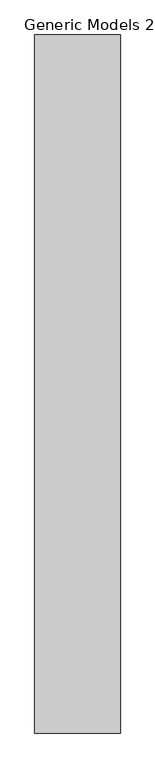
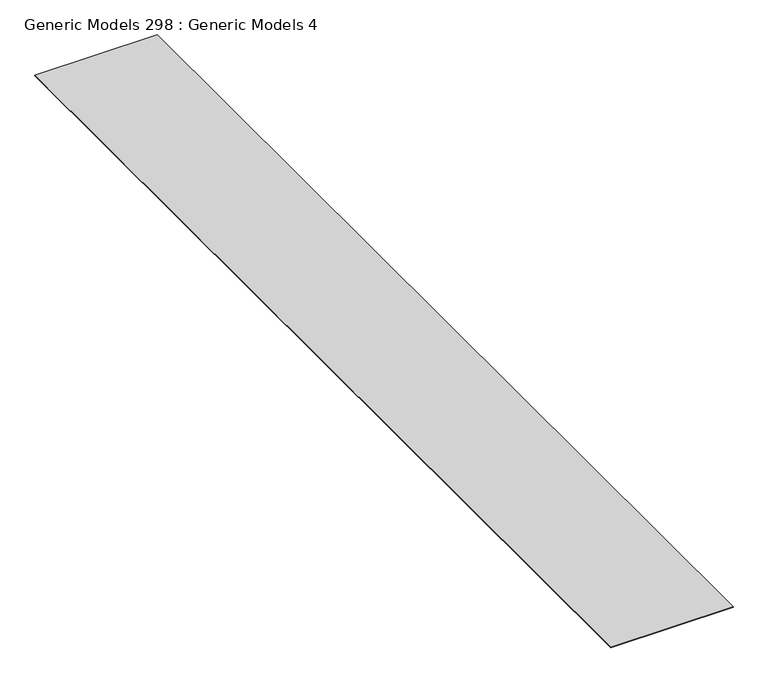
"""IFC4 building model written with IfcOpenShell, lengths in millimetres: proxy geometry, Generic Models 298 : Generic Models 4."""

import ifcopenshell
import ifcopenshell.guid

model = None  # the IFC model being written
_history = None  # IfcOwnerHistory: only IFC2X3 demands one
_inside = {}  # id of a spatial element -> (the spatial element, [elements in it])
_under = {}  # id of a project, library or spatial element -> (it, [spatial elements below it])
_declared = {}  # id of a project -> (the project, [libraries it declares])
_typed = {}  # id of a type object -> (the type object, [elements of that type])
_made_of = {}  # id of a material, layer set ... -> (it, [elements and type objects made of it])


def new_model(schema):
    """Start an empty IFC model of exactly this schema.

    Asked for "IFC4X3", IfcOpenShell would pick the latest addendum, in which some entities
    have other attributes; the version numbers below select the first issue.
    IFC2X3 requires an IfcOwnerHistory on every rooted entity: one is made here for all.
    """
    global model, _history
    if schema == "IFC4X3":
        model = ifcopenshell.file(schema_version=(4, 3, 0, 0))
    else:
        model = ifcopenshell.file(schema=schema)
    _inside.clear()
    _under.clear()
    _declared.clear()
    _typed.clear()
    _made_of.clear()
    _history = None
    if model.schema == "IFC2X3":
        org = make("IfcOrganization", Name="unknown")
        user = make(
            "IfcPersonAndOrganization",
            ThePerson=make("IfcPerson", FamilyName="unknown"),
            TheOrganization=org,
        )
        app = make(
            "IfcApplication",
            ApplicationDeveloper=org,
            Version="unknown",
            ApplicationFullName="unknown",
            ApplicationIdentifier="unknown",
        )
        _history = make(
            "IfcOwnerHistory",
            OwningUser=user,
            OwningApplication=app,
            ChangeAction="ADDED",
            CreationDate=0,
        )
    return model


def make(cls, **values):
    """One entity of the class cls with the attributes given. An attribute that is None is left unset."""
    return model.create_entity(
        cls, **{name: value for name, value in values.items() if value is not None}
    )


def rooted(cls, **values):
    """An entity with a GlobalId (a new one), such as an element, a storey or a relation."""
    return make(cls, GlobalId=ifcopenshell.guid.new(), OwnerHistory=_history, **values)


def si_unit(unit_type, name, prefix=None):
    """IfcSIUnit, for example si_unit("LENGTHUNIT", "METRE", prefix="MILLI")."""
    return make("IfcSIUnit", UnitType=unit_type, Prefix=prefix, Name=name)


def assignment(units):
    """IfcUnitAssignment: the units of a project."""
    return None if units is None else make("IfcUnitAssignment", Units=units)


def point(xyz):
    """IfcCartesianPoint."""
    return None if xyz is None else make("IfcCartesianPoint", Coordinates=xyz)


def direction(xyz):
    """IfcDirection."""
    return None if xyz is None else make("IfcDirection", DirectionRatios=xyz)


def frame(location, z_axis=None, x_axis=None):
    """IfcAxis2Placement3D, a coordinate frame: its origin and axes. An axis left out is left unset."""
    return make(
        "IfcAxis2Placement3D",
        Location=point(location),
        Axis=direction(z_axis),
        RefDirection=direction(x_axis),
    )


def origin():
    """The frame at (0, 0, 0) with its axes left unset."""
    return frame((0.0, 0.0, 0.0))


def place(relative_to, where):
    """IfcLocalPlacement: puts the frame where relative to a parent placement (None: the world)."""
    return make(
        "IfcLocalPlacement", PlacementRelTo=relative_to, RelativePlacement=where
    )


def context(
    kind, dimensions, precision=None, world=None, true_north=None, identifier=None
):
    """IfcGeometricRepresentationContext, for example the 3D "Model" context."""
    return make(
        "IfcGeometricRepresentationContext",
        ContextIdentifier=identifier,
        ContextType=kind,
        CoordinateSpaceDimension=dimensions,
        Precision=precision,
        WorldCoordinateSystem=world,
        TrueNorth=true_north,
    )


def project(units=None, contexts=None):
    """IfcProject with its units and contexts."""
    return rooted(
        "IfcProject",
        Name="project",
        RepresentationContexts=contexts,
        UnitsInContext=assignment(units),
    )


def spatial(cls, under=None, at=None, **own):
    """A site, building, storey or space (cls), placed at a placement, below another one or the project."""
    s = rooted(cls, ObjectPlacement=at, **own)
    if under is not None:
        _under.setdefault(under.id(), (under, []))[1].append(s)
    return s


def polyline(points):
    """IfcPolyline through the points."""
    return make("IfcPolyline", Points=[point(p) for p in points])


def outline(outer, holes=None, kind="AREA"):
    """IfcArbitraryClosedProfileDef: a profile drawn as a closed curve; with holes, ...WithVoids."""
    if holes is None:
        return make("IfcArbitraryClosedProfileDef", ProfileType=kind, OuterCurve=outer)
    return make(
        "IfcArbitraryProfileDefWithVoids",
        ProfileType=kind,
        OuterCurve=outer,
        InnerCurves=holes,
    )


def extrude(swept, where, along, depth):
    """IfcExtrudedAreaSolid: the profile swept, set in the frame where, extruded along a direction by depth."""
    return make(
        "IfcExtrudedAreaSolid",
        SweptArea=swept,
        Position=where,
        ExtrudedDirection=direction(along),
        Depth=depth,
    )


def shape(context_of_items, identifier, shape_type, items):
    """IfcShapeRepresentation: the items that make up one representation, for example the "Body"."""
    return make(
        "IfcShapeRepresentation",
        ContextOfItems=context_of_items,
        RepresentationIdentifier=identifier,
        RepresentationType=shape_type,
        Items=items,
    )


def source(mapping_origin, context_of_items, identifier, shape_type, items):
    """IfcRepresentationMap: a shape defined once, which mapped items show again and again."""
    return make(
        "IfcRepresentationMap",
        MappingOrigin=mapping_origin,
        MappedRepresentation=shape(context_of_items, identifier, shape_type, items),
    )


def transform(
    local_origin,
    x_axis=None,
    y_axis=None,
    z_axis=None,
    scale=None,
    scale2=None,
    scale3=None,
    uniform=True,
):
    """IfcCartesianTransformationOperator3D, or its non-uniform kind. x_axis, y_axis, z_axis: its Axis1, 2, 3."""
    if uniform:
        return make(
            "IfcCartesianTransformationOperator3D",
            Axis1=direction(x_axis),
            Axis2=direction(y_axis),
            LocalOrigin=point(local_origin),
            Scale=scale,
            Axis3=direction(z_axis),
        )
    return make(
        "IfcCartesianTransformationOperator3DnonUniform",
        Axis1=direction(x_axis),
        Axis2=direction(y_axis),
        LocalOrigin=point(local_origin),
        Scale=scale,
        Axis3=direction(z_axis),
        Scale2=scale2,
        Scale3=scale3,
    )


def mapped(mapping_source, mapping_target):
    """IfcMappedItem: shows the shape of a source again, moved by a transform."""
    return make(
        "IfcMappedItem", MappingSource=mapping_source, MappingTarget=mapping_target
    )


def made_of(thing, what):
    """Note that an element or type object is made of a material, layer set ...; save() writes the relation."""
    if what is not None:
        _made_of.setdefault(what.id(), (what, []))[1].append(thing)
    return thing


def element(
    cls,
    number,
    at=None,
    inside=None,
    cuts=None,
    type_object=None,
    material=None,
    context=None,
    identifier="Body",
    shape_type=None,
    held_by="IfcProductDefinitionShape",
    body=None,
    shapes=None,
    **own,
):
    """One element of the class cls, such as IfcWall. Its Tag is "e" and its number.

    at: its placement. inside: the storey or other place that contains it. cuts: it is an
    opening in that element (IfcRelVoidsElement). A single representation is given by context,
    identifier, shape_type and body (its items); several are given by shapes. held_by: the class
    of the entity that holds the representations. save() writes the other relations.
    """
    e = rooted(cls, Tag="e%d" % number, ObjectPlacement=at, **own)
    if body is not None:
        shapes = [shape(context, identifier, shape_type, body)]
    if shapes is not None:
        e.Representation = make(held_by, Representations=shapes)
    if inside is not None:
        _inside.setdefault(inside.id(), (inside, []))[1].append(e)
    if cuts is not None:
        rooted(
            "IfcRelVoidsElement", RelatingBuildingElement=cuts, RelatedOpeningElement=e
        )
    if type_object is not None:
        _typed.setdefault(type_object.id(), (type_object, []))[1].append(e)
    return made_of(e, material)


def aggregate(whole, parts):
    """IfcRelAggregates: a whole, such as a stair, and the parts it consists of."""
    return rooted("IfcRelAggregates", RelatingObject=whole, RelatedObjects=parts)


def save(model, path):
    """Write the relations noted so far, then the file.

    IfcRelAggregates (storeys below a building ...), IfcRelContainedInSpatialStructure (elements
    in a storey), IfcRelDefinesByType, IfcRelAssociatesMaterial and IfcRelDeclares: one each for
    every whole, place, type object, material and project.
    """
    for whole, parts in _under.values():
        aggregate(whole, parts)
    for where, things in _inside.values():
        rooted(
            "IfcRelContainedInSpatialStructure",
            RelatedElements=things,
            RelatingStructure=where,
        )
    for kind, things in _typed.values():
        rooted("IfcRelDefinesByType", RelatedObjects=things, RelatingType=kind)
    for what, things in _made_of.values():
        rooted("IfcRelAssociatesMaterial", RelatedObjects=things, RelatingMaterial=what)
    for by, libraries in _declared.values():
        rooted("IfcRelDeclares", RelatingContext=by, RelatedDefinitions=libraries)
    model.write(path)


def generic_models_298_generic_models_4_816b7251(model_context):
    return source(origin(), model_context, "Body", "SweptSolid", [
        extrude(outline(polyline([(-5950.1236296, 2583.8769662), (-6498.6122941, 2583.8769662), (-6498.6122941, 7054.2769662), (-5950.1236296, 7054.2769662), (-5950.1236296, 2583.8769662)])), frame((0.0, 0.0, 123259.596), z_axis=(0.0, 0.0, 1.0), x_axis=(1.0, 0.0, 0.0)), (0.0, 0.0, 1.0), 1.5875),
    ])


if __name__ == "__main__":
    model = new_model("IFC4")
    model_context = context("Model", 3, world=origin())
    ifc_project = project(units=[si_unit("LENGTHUNIT", "METRE", prefix="MILLI")], contexts=[model_context])
    site = spatial("IfcSite", under=ifc_project)
    building = spatial("IfcBuilding", under=site)
    placement = place(None, origin())
    generic_models_298_generic_models_4_shape = generic_models_298_generic_models_4_816b7251(model_context)
    element("IfcBuildingElementProxy", 1, Name="Generic Models 298 : Generic Models 4", ObjectType="Generic Models 298 : Generic Models 4", at=placement, inside=building, context=model_context, shape_type="MappedRepresentation", body=[
        mapped(generic_models_298_generic_models_4_shape, transform((0.0, 0.0, 0.0), x_axis=(1.0, 0.0, 0.0), y_axis=(0.0, 1.0, 0.0), z_axis=(0.0, 0.0, 1.0))),
    ])
    save(model, "model.ifc")

# Revit data of these elements
# Element 1 (IfcBuildingElementProxy, "Generic Models 298 : Generic Models 4")
#   Materials on its faces: "_6 MIL VAPOR BARRIER"
# Materials
#   "_6 MIL VAPOR BARRIER": class "Generic", colour RGB 67 154 161, transparency 0, Cost = 0
